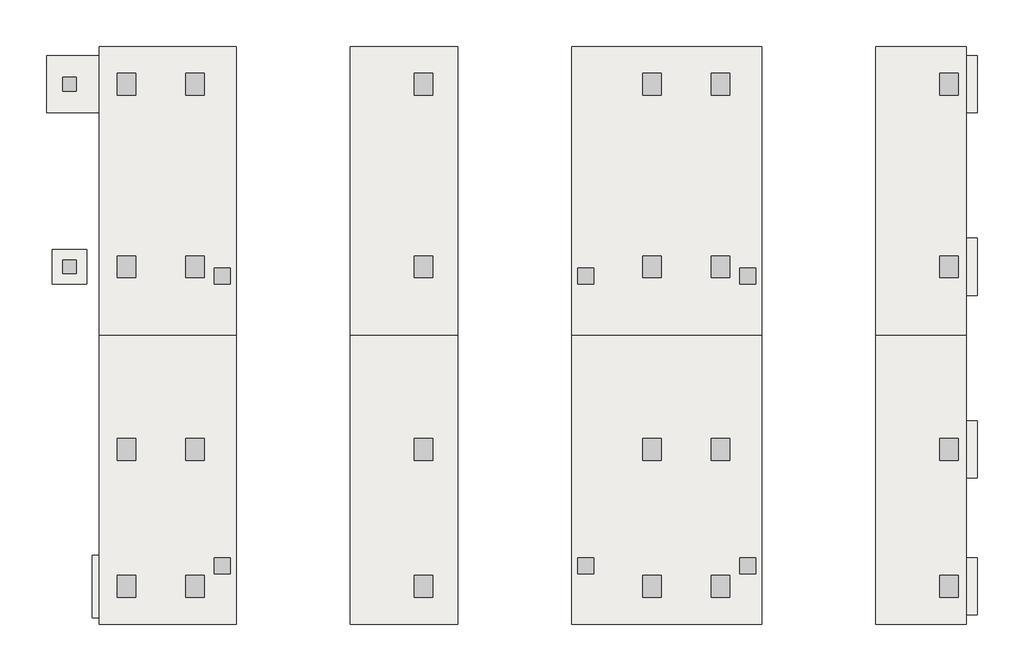
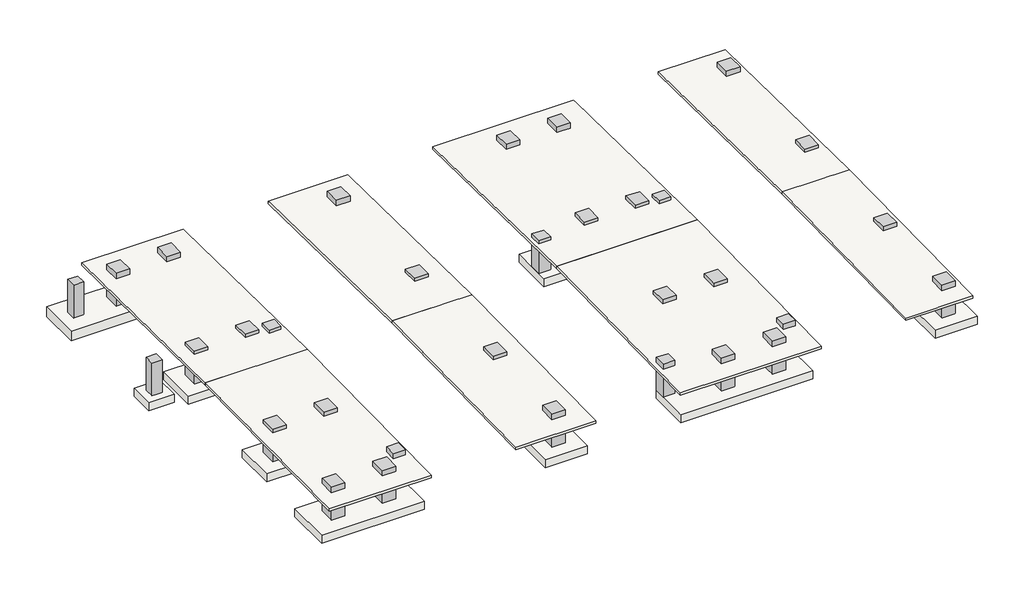
# Not in any storey: 32 columns, 25 slabs.
"""IFC4 building model written with IfcOpenShell, lengths in millimetres."""

import ifcopenshell
import ifcopenshell.guid

model = None  # the IFC model being written
_history = None  # IfcOwnerHistory: only IFC2X3 demands one
_inside = {}  # id of a spatial element -> (the spatial element, [elements in it])
_under = {}  # id of a project, library or spatial element -> (it, [spatial elements below it])
_declared = {}  # id of a project -> (the project, [libraries it declares])
_typed = {}  # id of a type object -> (the type object, [elements of that type])
_made_of = {}  # id of a material, layer set ... -> (it, [elements and type objects made of it])


def new_model(schema):
    """Start an empty IFC model of exactly this schema.

    Asked for "IFC4X3", IfcOpenShell would pick the latest addendum, in which some entities
    have other attributes; the version numbers below select the first issue.
    IFC2X3 requires an IfcOwnerHistory on every rooted entity: one is made here for all.
    """
    global model, _history
    if schema == "IFC4X3":
        model = ifcopenshell.file(schema_version=(4, 3, 0, 0))
    else:
        model = ifcopenshell.file(schema=schema)
    _inside.clear()
    _under.clear()
    _declared.clear()
    _typed.clear()
    _made_of.clear()
    _history = None
    if model.schema == "IFC2X3":
        org = make("IfcOrganization", Name="unknown")
        user = make(
            "IfcPersonAndOrganization",
            ThePerson=make("IfcPerson", FamilyName="unknown"),
            TheOrganization=org,
        )
        app = make(
            "IfcApplication",
            ApplicationDeveloper=org,
            Version="unknown",
            ApplicationFullName="unknown",
            ApplicationIdentifier="unknown",
        )
        _history = make(
            "IfcOwnerHistory",
            OwningUser=user,
            OwningApplication=app,
            ChangeAction="ADDED",
            CreationDate=0,
        )
    return model


def make(cls, **values):
    """One entity of the class cls with the attributes given. An attribute that is None is left unset."""
    return model.create_entity(
        cls, **{name: value for name, value in values.items() if value is not None}
    )


def rooted(cls, **values):
    """An entity with a GlobalId (a new one), such as an element, a storey or a relation."""
    return make(cls, GlobalId=ifcopenshell.guid.new(), OwnerHistory=_history, **values)


def si_unit(unit_type, name, prefix=None):
    """IfcSIUnit, for example si_unit("LENGTHUNIT", "METRE", prefix="MILLI")."""
    return make("IfcSIUnit", UnitType=unit_type, Prefix=prefix, Name=name)


def assignment(units):
    """IfcUnitAssignment: the units of a project."""
    return None if units is None else make("IfcUnitAssignment", Units=units)


def point(xyz):
    """IfcCartesianPoint."""
    return None if xyz is None else make("IfcCartesianPoint", Coordinates=xyz)


def direction(xyz):
    """IfcDirection."""
    return None if xyz is None else make("IfcDirection", DirectionRatios=xyz)


def frame(location, z_axis=None, x_axis=None):
    """IfcAxis2Placement3D, a coordinate frame: its origin and axes. An axis left out is left unset."""
    return make(
        "IfcAxis2Placement3D",
        Location=point(location),
        Axis=direction(z_axis),
        RefDirection=direction(x_axis),
    )


def origin():
    """The frame at (0, 0, 0) with its axes left unset."""
    return frame((0.0, 0.0, 0.0))


def place(relative_to, where):
    """IfcLocalPlacement: puts the frame where relative to a parent placement (None: the world)."""
    return make(
        "IfcLocalPlacement", PlacementRelTo=relative_to, RelativePlacement=where
    )


def context(
    kind, dimensions, precision=None, world=None, true_north=None, identifier=None
):
    """IfcGeometricRepresentationContext, for example the 3D "Model" context."""
    return make(
        "IfcGeometricRepresentationContext",
        ContextIdentifier=identifier,
        ContextType=kind,
        CoordinateSpaceDimension=dimensions,
        Precision=precision,
        WorldCoordinateSystem=world,
        TrueNorth=true_north,
    )


def project(units=None, contexts=None):
    """IfcProject with its units and contexts."""
    return rooted(
        "IfcProject",
        Name="project",
        RepresentationContexts=contexts,
        UnitsInContext=assignment(units),
    )


def spatial(cls, under=None, at=None, **own):
    """A site, building, storey or space (cls), placed at a placement, below another one or the project."""
    s = rooted(cls, ObjectPlacement=at, **own)
    if under is not None:
        _under.setdefault(under.id(), (under, []))[1].append(s)
    return s


def polyline(points):
    """IfcPolyline through the points."""
    return make("IfcPolyline", Points=[point(p) for p in points])


def outline(outer, holes=None, kind="AREA"):
    """IfcArbitraryClosedProfileDef: a profile drawn as a closed curve; with holes, ...WithVoids."""
    if holes is None:
        return make("IfcArbitraryClosedProfileDef", ProfileType=kind, OuterCurve=outer)
    return make(
        "IfcArbitraryProfileDefWithVoids",
        ProfileType=kind,
        OuterCurve=outer,
        InnerCurves=holes,
    )


def extrude(swept, where, along, depth):
    """IfcExtrudedAreaSolid: the profile swept, set in the frame where, extruded along a direction by depth."""
    return make(
        "IfcExtrudedAreaSolid",
        SweptArea=swept,
        Position=where,
        ExtrudedDirection=direction(along),
        Depth=depth,
    )


def faces_of(points, faces, orient=None, outer=None):
    """IfcFace entities. A face is a list of loops; a loop is a list of indices into points, from 0.

    orient and outer hold one flag for each loop. By default every Orientation is true, the
    first loop of a face is its IfcFaceOuterBound and the others are IfcFaceBound.
    """
    made = []
    for i, loops in enumerate(faces):
        bounds = []
        for j, loop in enumerate(loops):
            is_outer = j == 0 if outer is None else outer[i][j]
            bounds.append(
                make(
                    "IfcFaceOuterBound" if is_outer else "IfcFaceBound",
                    Bound=make("IfcPolyLoop", Polygon=[points[k] for k in loop]),
                    Orientation=True if orient is None else orient[i][j],
                )
            )
        made.append(make("IfcFace", Bounds=bounds))
    return made


def faceted_brep(points, faces, orient=None, outer=None, voids=None):
    """IfcFacetedBrep: a solid bounded by flat faces; with voids (closed shells), ...WithVoids."""
    shared = [point(p) for p in points]
    hull = make("IfcClosedShell", CfsFaces=faces_of(shared, faces, orient, outer))
    if voids is None:
        return make("IfcFacetedBrep", Outer=hull)
    return make(
        "IfcFacetedBrepWithVoids",
        Outer=hull,
        Voids=[
            make(cls, CfsFaces=faces_of(shared, fs, o, b)) for cls, fs, o, b in voids
        ],
    )


def shape(context_of_items, identifier, shape_type, items):
    """IfcShapeRepresentation: the items that make up one representation, for example the "Body"."""
    return make(
        "IfcShapeRepresentation",
        ContextOfItems=context_of_items,
        RepresentationIdentifier=identifier,
        RepresentationType=shape_type,
        Items=items,
    )


def source(mapping_origin, context_of_items, identifier, shape_type, items):
    """IfcRepresentationMap: a shape defined once, which mapped items show again and again."""
    return make(
        "IfcRepresentationMap",
        MappingOrigin=mapping_origin,
        MappedRepresentation=shape(context_of_items, identifier, shape_type, items),
    )


def transform(
    local_origin,
    x_axis=None,
    y_axis=None,
    z_axis=None,
    scale=None,
    scale2=None,
    scale3=None,
    uniform=True,
):
    """IfcCartesianTransformationOperator3D, or its non-uniform kind. x_axis, y_axis, z_axis: its Axis1, 2, 3."""
    if uniform:
        return make(
            "IfcCartesianTransformationOperator3D",
            Axis1=direction(x_axis),
            Axis2=direction(y_axis),
            LocalOrigin=point(local_origin),
            Scale=scale,
            Axis3=direction(z_axis),
        )
    return make(
        "IfcCartesianTransformationOperator3DnonUniform",
        Axis1=direction(x_axis),
        Axis2=direction(y_axis),
        LocalOrigin=point(local_origin),
        Scale=scale,
        Axis3=direction(z_axis),
        Scale2=scale2,
        Scale3=scale3,
    )


def mapped(mapping_source, mapping_target):
    """IfcMappedItem: shows the shape of a source again, moved by a transform."""
    return make(
        "IfcMappedItem", MappingSource=mapping_source, MappingTarget=mapping_target
    )


def made_of(thing, what):
    """Note that an element or type object is made of a material, layer set ...; save() writes the relation."""
    if what is not None:
        _made_of.setdefault(what.id(), (what, []))[1].append(thing)
    return thing


def element(
    cls,
    number,
    at=None,
    inside=None,
    cuts=None,
    type_object=None,
    material=None,
    context=None,
    identifier="Body",
    shape_type=None,
    held_by="IfcProductDefinitionShape",
    body=None,
    shapes=None,
    **own,
):
    """One element of the class cls, such as IfcWall. Its Tag is "e" and its number.

    at: its placement. inside: the storey or other place that contains it. cuts: it is an
    opening in that element (IfcRelVoidsElement). A single representation is given by context,
    identifier, shape_type and body (its items); several are given by shapes. held_by: the class
    of the entity that holds the representations. save() writes the other relations.
    """
    e = rooted(cls, Tag="e%d" % number, ObjectPlacement=at, **own)
    if body is not None:
        shapes = [shape(context, identifier, shape_type, body)]
    if shapes is not None:
        e.Representation = make(held_by, Representations=shapes)
    if inside is not None:
        _inside.setdefault(inside.id(), (inside, []))[1].append(e)
    if cuts is not None:
        rooted(
            "IfcRelVoidsElement", RelatingBuildingElement=cuts, RelatedOpeningElement=e
        )
    if type_object is not None:
        _typed.setdefault(type_object.id(), (type_object, []))[1].append(e)
    return made_of(e, material)


def aggregate(whole, parts):
    """IfcRelAggregates: a whole, such as a stair, and the parts it consists of."""
    return rooted("IfcRelAggregates", RelatingObject=whole, RelatedObjects=parts)


def save(model, path):
    """Write the relations noted so far, then the file.

    IfcRelAggregates (storeys below a building ...), IfcRelContainedInSpatialStructure (elements
    in a storey), IfcRelDefinesByType, IfcRelAssociatesMaterial and IfcRelDeclares: one each for
    every whole, place, type object, material and project.
    """
    for whole, parts in _under.values():
        aggregate(whole, parts)
    for where, things in _inside.values():
        rooted(
            "IfcRelContainedInSpatialStructure",
            RelatedElements=things,
            RelatingStructure=where,
        )
    for kind, things in _typed.values():
        rooted("IfcRelDefinesByType", RelatedObjects=things, RelatingType=kind)
    for what, things in _made_of.values():
        rooted("IfcRelAssociatesMaterial", RelatedObjects=things, RelatingMaterial=what)
    for by, libraries in _declared.values():
        rooted("IfcRelDeclares", RelatingContext=by, RelatedDefinitions=libraries)
    model.write(path)


def rc_column_rectangular_8fcc3407(model_context):
    return source(origin(), model_context, "Body", "SweptSolid", [
        extrude(outline(polyline([(400.0, 475.0), (400.0, -475.0), (-400.0, -475.0), (-400.0, 475.0), (400.0, 475.0)])), frame((0.0, 0.0, -9380.1756499), z_axis=(0.0, 0.0, 1.0), x_axis=(1.0, 0.0, 0.0)), (0.0, 0.0, 1.0), 2050.0),
    ])


def rc_column_rectangular_fa199b6f(model_context):
    return source(origin(), model_context, "Body", "SweptSolid", [
        extrude(outline(polyline([(300.0, 300.0), (300.0, -300.0), (-300.0, -300.0), (-300.0, 300.0), (300.0, 300.0)])), frame((0.0, 0.0, -9380.1756499), z_axis=(0.0, 0.0, 1.0), x_axis=(1.0, 0.0, 0.0)), (0.0, 0.0, 1.0), 2050.0),
    ])


def rc_column_rectangular_f0532c4b(model_context):
    return source(origin(), model_context, "Body", "SweptSolid", [
        extrude(outline(polyline([(350.0, 350.0), (350.0, -350.0), (-350.0, -350.0), (-350.0, 350.0), (350.0, 350.0)])), frame((0.0, 0.0, -9380.1756499), z_axis=(0.0, 0.0, 1.0), x_axis=(1.0, 0.0, 0.0)), (0.0, 0.0, 1.0), 2050.0),
    ])


def footing_rectangular_r1_513089b3(model_context):
    return source(origin(), model_context, "Body", "SweptSolid", [
        extrude(outline(polyline([(1250.0, 1250.0), (1250.0, -1250.0), (-1250.0, -1250.0), (-1250.0, 1250.0), (1250.0, 1250.0)])), frame((0.0, 0.0, -500.0), z_axis=(0.0, 0.0, 1.0), x_axis=(1.0, 0.0, 0.0)), (0.0, 0.0, 1.0), 500.0),
    ])


def footing_rectangular_r1_601d9235(model_context):
    return source(origin(), model_context, "Body", "SweptSolid", [
        extrude(outline(polyline([(750.0, 750.0), (750.0, -750.0), (-750.0, -750.0), (-750.0, 750.0), (750.0, 750.0)])), frame((0.0, 0.0, -500.0), z_axis=(0.0, 0.0, 1.0), x_axis=(1.0, 0.0, 0.0)), (0.0, 0.0, 1.0), 500.0),
    ])


def footing_rectangular_r1_ca059662(model_context):
    return source(origin(), model_context, "Body", "SweptSolid", [
        extrude(outline(polyline([(2700.0, 1250.0), (2700.0, -1250.0), (-2700.0, -1250.0), (-2700.0, 1250.0), (2700.0, 1250.0)])), frame((0.0, 0.0, -500.0), z_axis=(0.0, 0.0, 1.0), x_axis=(1.0, 0.0, 0.0)), (0.0, 0.0, 1.0), 500.0),
    ])


def footing_rectangular_r1_297981ed(model_context):
    return source(origin(), model_context, "Body", "SweptSolid", [
        extrude(outline(polyline([(3000.0, 1250.0), (3000.0, -1250.0), (-3000.0, -1250.0), (-3000.0, 1250.0), (3000.0, 1250.0)])), frame((0.0, 0.0, -500.0), z_axis=(0.0, 0.0, 1.0), x_axis=(1.0, 0.0, 0.0)), (0.0, 0.0, 1.0), 500.0),
    ])


def footing_rectangular_r1_282b4f06(model_context):
    return source(origin(), model_context, "Body", "SweptSolid", [
        extrude(outline(polyline([(4000.0, 1250.0), (4000.0, -1250.0), (-4000.0, -1250.0), (-4000.0, 1250.0), (4000.0, 1250.0)])), frame((0.0, 0.0, -600.0), z_axis=(0.0, 0.0, 1.0), x_axis=(1.0, 0.0, 0.0)), (0.0, 0.0, 1.0), 600.0),
    ])


def footing_rectangular_r1_f7e30f5b(model_context):
    return source(origin(), model_context, "Body", "SweptSolid", [
        extrude(outline(polyline([(2875.0, 1250.0), (2875.0, -1250.0), (-2875.0, -1250.0), (-2875.0, 1250.0), (2875.0, 1250.0)])), frame((0.0, 0.0, -500.0), z_axis=(0.0, 0.0, 1.0), x_axis=(1.0, 0.0, 0.0)), (0.0, 0.0, 1.0), 500.0),
    ])


def footing_rectangular_r1_e1557040(model_context):
    return source(origin(), model_context, "Body", "SweptSolid", [
        extrude(outline(polyline([(3900.0, 1250.0), (3900.0, -1250.0), (-3900.0, -1250.0), (-3900.0, 1250.0), (3900.0, 1250.0)])), frame((0.0, 0.0, -500.0), z_axis=(0.0, 0.0, 1.0), x_axis=(1.0, 0.0, 0.0)), (0.0, 0.0, 1.0), 500.0),
    ])


def footing_rectangular_r1_8e80394c(model_context):
    return source(origin(), model_context, "Body", "SweptSolid", [
        extrude(outline(polyline([(3025.0, 1370.0), (3025.0, -1370.0), (-3025.0, -1370.0), (-3025.0, 1370.0), (3025.0, 1370.0)])), frame((0.0, 0.0, -500.0), z_axis=(0.0, 0.0, 1.0), x_axis=(1.0, 0.0, 0.0)), (0.0, 0.0, 1.0), 500.0),
    ])


model = new_model("IFC4")

# Units and contexts
model_context = context("Model", 3, world=origin())
ifc_project = project(units=[si_unit("LENGTHUNIT", "METRE", prefix="MILLI")], contexts=[model_context])

# Site, building
site = spatial("IfcSite", under=ifc_project)
building = spatial("IfcBuilding", under=site)

# Columns
placement = place(None, origin())
rc_column_rectangular_shape = rc_column_rectangular_8fcc3407(model_context)
element("IfcColumn", 1, ObjectType="RC_Column_Rectangular : H_SC_AR_S15_UG PED_W800xL950_Bit_PD1", at=placement, inside=building, context=model_context, shape_type="MappedRepresentation", body=[
    mapped(rc_column_rectangular_shape, transform((36000.0, 499.5208589, 0.0), x_axis=(1.0, 0.0, 0.0), y_axis=(0.0, 1.0, 0.0), z_axis=(0.0, 0.0, 1.0))),
])
element("IfcColumn", 2, ObjectType="RC_Column_Rectangular : H_SC_AR_S15_UG PED_W800xL950_Bit_PD1", at=placement, inside=building, context=model_context, shape_type="MappedRepresentation", body=[
    mapped(rc_column_rectangular_shape, transform((36000.0, 6499.5208589, 0.0), x_axis=(1.0, 0.0, 0.0), y_axis=(0.0, 1.0, 0.0), z_axis=(0.0, 0.0, 1.0))),
])
element("IfcColumn", 3, ObjectType="RC_Column_Rectangular : H_SC_AR_S15_UG PED_W800xL950_Bit_PD1", at=placement, inside=building, context=model_context, shape_type="MappedRepresentation", body=[
    mapped(rc_column_rectangular_shape, transform((36000.0, 14499.5208589, 0.0), x_axis=(1.0, 0.0, 0.0), y_axis=(0.0, 1.0, 0.0), z_axis=(0.0, 0.0, 1.0))),
])
element("IfcColumn", 4, ObjectType="RC_Column_Rectangular : H_SC_AR_S15_UG PED_W800xL950_Bit_PD1", at=placement, inside=building, context=model_context, shape_type="MappedRepresentation", body=[
    mapped(rc_column_rectangular_shape, transform((36000.0, 22499.5208589, 0.0), x_axis=(1.0, 0.0, 0.0), y_axis=(0.0, 1.0, 0.0), z_axis=(0.0, 0.0, 1.0))),
])
element("IfcColumn", 5, ObjectType="RC_Column_Rectangular : H_SC_AR_S15_UG PED_W800xL950_Bit_PD1", at=placement, inside=building, context=model_context, shape_type="MappedRepresentation", body=[
    mapped(rc_column_rectangular_shape, transform((26000.0, 499.5208589, 0.0), x_axis=(1.0, 0.0, 0.0), y_axis=(0.0, 1.0, 0.0), z_axis=(0.0, 0.0, 1.0))),
])
element("IfcColumn", 6, ObjectType="RC_Column_Rectangular : H_SC_AR_S15_UG PED_W800xL950_Bit_PD1", at=placement, inside=building, context=model_context, shape_type="MappedRepresentation", body=[
    mapped(rc_column_rectangular_shape, transform((26000.0, 6499.5208589, 0.0), x_axis=(1.0, 0.0, 0.0), y_axis=(0.0, 1.0, 0.0), z_axis=(0.0, 0.0, 1.0))),
])
element("IfcColumn", 7, ObjectType="RC_Column_Rectangular : H_SC_AR_S15_UG PED_W800xL950_Bit_PD1", at=placement, inside=building, context=model_context, shape_type="MappedRepresentation", body=[
    mapped(rc_column_rectangular_shape, transform((26000.0, 14499.5208589, 0.0), x_axis=(1.0, 0.0, 0.0), y_axis=(0.0, 1.0, 0.0), z_axis=(0.0, 0.0, 1.0))),
])
element("IfcColumn", 8, ObjectType="RC_Column_Rectangular : H_SC_AR_S15_UG PED_W800xL950_Bit_PD1", at=placement, inside=building, context=model_context, shape_type="MappedRepresentation", body=[
    mapped(rc_column_rectangular_shape, transform((26000.0, 22499.5208589, 0.0), x_axis=(1.0, 0.0, 0.0), y_axis=(0.0, 1.0, 0.0), z_axis=(0.0, 0.0, 1.0))),
])
element("IfcColumn", 9, ObjectType="RC_Column_Rectangular : H_SC_AR_S15_UG PED_W800xL950_Bit_PD1", at=placement, inside=building, context=model_context, shape_type="MappedRepresentation", body=[
    mapped(rc_column_rectangular_shape, transform((23000.0, 499.5208589, 0.0), x_axis=(1.0, 0.0, 0.0), y_axis=(0.0, 1.0, 0.0), z_axis=(0.0, 0.0, 1.0))),
])
element("IfcColumn", 10, ObjectType="RC_Column_Rectangular : H_SC_AR_S15_UG PED_W800xL950_Bit_PD1", at=placement, inside=building, context=model_context, shape_type="MappedRepresentation", body=[
    mapped(rc_column_rectangular_shape, transform((23000.0, 6499.5208589, 0.0), x_axis=(1.0, 0.0, 0.0), y_axis=(0.0, 1.0, 0.0), z_axis=(0.0, 0.0, 1.0))),
])
element("IfcColumn", 11, ObjectType="RC_Column_Rectangular : H_SC_AR_S15_UG PED_W800xL950_Bit_PD1", at=placement, inside=building, context=model_context, shape_type="MappedRepresentation", body=[
    mapped(rc_column_rectangular_shape, transform((23000.0, 14499.5208589, 0.0), x_axis=(1.0, 0.0, 0.0), y_axis=(0.0, 1.0, 0.0), z_axis=(0.0, 0.0, 1.0))),
])
element("IfcColumn", 12, ObjectType="RC_Column_Rectangular : H_SC_AR_S15_UG PED_W800xL950_Bit_PD1", at=placement, inside=building, context=model_context, shape_type="MappedRepresentation", body=[
    mapped(rc_column_rectangular_shape, transform((23000.0, 22499.5208589, 0.0), x_axis=(1.0, 0.0, 0.0), y_axis=(0.0, 1.0, 0.0), z_axis=(0.0, 0.0, 1.0))),
])
element("IfcColumn", 13, ObjectType="RC_Column_Rectangular : H_SC_AR_S15_UG PED_W800xL950_Bit_PD1", at=placement, inside=building, context=model_context, shape_type="MappedRepresentation", body=[
    mapped(rc_column_rectangular_shape, transform((13000.0, 499.5208589, 0.0), x_axis=(1.0, 0.0, 0.0), y_axis=(0.0, 1.0, 0.0), z_axis=(0.0, 0.0, 1.0))),
])
element("IfcColumn", 14, ObjectType="RC_Column_Rectangular : H_SC_AR_S15_UG PED_W800xL950_Bit_PD1", at=placement, inside=building, context=model_context, shape_type="MappedRepresentation", body=[
    mapped(rc_column_rectangular_shape, transform((13000.0, 6499.5208589, 0.0), x_axis=(1.0, 0.0, 0.0), y_axis=(0.0, 1.0, 0.0), z_axis=(0.0, 0.0, 1.0))),
])
element("IfcColumn", 15, ObjectType="RC_Column_Rectangular : H_SC_AR_S15_UG PED_W800xL950_Bit_PD1", at=placement, inside=building, context=model_context, shape_type="MappedRepresentation", body=[
    mapped(rc_column_rectangular_shape, transform((13000.0, 14499.5208589, 0.0), x_axis=(1.0, 0.0, 0.0), y_axis=(0.0, 1.0, 0.0), z_axis=(0.0, 0.0, 1.0))),
])
element("IfcColumn", 16, ObjectType="RC_Column_Rectangular : H_SC_AR_S15_UG PED_W800xL950_Bit_PD1", at=placement, inside=building, context=model_context, shape_type="MappedRepresentation", body=[
    mapped(rc_column_rectangular_shape, transform((13000.0, 22499.5208589, 0.0), x_axis=(1.0, 0.0, 0.0), y_axis=(0.0, 1.0, 0.0), z_axis=(0.0, 0.0, 1.0))),
])
element("IfcColumn", 17, ObjectType="RC_Column_Rectangular : H_SC_AR_S15_UG PED_W800xL950_Bit_PD1", at=placement, inside=building, context=model_context, shape_type="MappedRepresentation", body=[
    mapped(rc_column_rectangular_shape, transform((3000.0, 499.5208589, 0.0), x_axis=(1.0, 0.0, 0.0), y_axis=(0.0, 1.0, 0.0), z_axis=(0.0, 0.0, 1.0))),
])
element("IfcColumn", 18, ObjectType="RC_Column_Rectangular : H_SC_AR_S15_UG PED_W800xL950_Bit_PD1", at=placement, inside=building, context=model_context, shape_type="MappedRepresentation", body=[
    mapped(rc_column_rectangular_shape, transform((3000.0, 6499.5208589, 0.0), x_axis=(1.0, 0.0, 0.0), y_axis=(0.0, 1.0, 0.0), z_axis=(0.0, 0.0, 1.0))),
])
element("IfcColumn", 19, ObjectType="RC_Column_Rectangular : H_SC_AR_S15_UG PED_W800xL950_Bit_PD1", at=placement, inside=building, context=model_context, shape_type="MappedRepresentation", body=[
    mapped(rc_column_rectangular_shape, transform((3000.0, 14499.5208589, 0.0), x_axis=(1.0, 0.0, 0.0), y_axis=(0.0, 1.0, 0.0), z_axis=(0.0, 0.0, 1.0))),
])
element("IfcColumn", 20, ObjectType="RC_Column_Rectangular : H_SC_AR_S15_UG PED_W800xL950_Bit_PD1", at=placement, inside=building, context=model_context, shape_type="MappedRepresentation", body=[
    mapped(rc_column_rectangular_shape, transform((3000.0, 22499.5208589, 0.0), x_axis=(1.0, 0.0, 0.0), y_axis=(0.0, 1.0, 0.0), z_axis=(0.0, 0.0, 1.0))),
])
element("IfcColumn", 21, ObjectType="RC_Column_Rectangular : H_SC_AR_S15_UG PED_W800xL950_Bit_PD1", at=placement, inside=building, context=model_context, shape_type="MappedRepresentation", body=[
    mapped(rc_column_rectangular_shape, transform((0.0, 499.5208589, 0.0), x_axis=(1.0, 0.0, 0.0), y_axis=(0.0, 1.0, 0.0), z_axis=(0.0, 0.0, 1.0))),
])
element("IfcColumn", 22, ObjectType="RC_Column_Rectangular : H_SC_AR_S15_UG PED_W800xL950_Bit_PD1", at=placement, inside=building, context=model_context, shape_type="MappedRepresentation", body=[
    mapped(rc_column_rectangular_shape, transform((0.0, 6499.5208589, 0.0), x_axis=(1.0, 0.0, 0.0), y_axis=(0.0, 1.0, 0.0), z_axis=(0.0, 0.0, 1.0))),
])
element("IfcColumn", 23, ObjectType="RC_Column_Rectangular : H_SC_AR_S15_UG PED_W800xL950_Bit_PD1", at=placement, inside=building, context=model_context, shape_type="MappedRepresentation", body=[
    mapped(rc_column_rectangular_shape, transform((0.0, 14499.5208589, 0.0), x_axis=(1.0, 0.0, 0.0), y_axis=(0.0, 1.0, 0.0), z_axis=(0.0, 0.0, 1.0))),
])
element("IfcColumn", 24, ObjectType="RC_Column_Rectangular : H_SC_AR_S15_UG PED_W800xL950_Bit_PD1", at=placement, inside=building, context=model_context, shape_type="MappedRepresentation", body=[
    mapped(rc_column_rectangular_shape, transform((0.0, 22499.5208589, 0.0), x_axis=(1.0, 0.0, 0.0), y_axis=(0.0, 1.0, 0.0), z_axis=(0.0, 0.0, 1.0))),
])
rc_column_rectangular_2_shape = rc_column_rectangular_fa199b6f(model_context)
element("IfcColumn", 25, ObjectType="RC_Column_Rectangular : H_SC_AR_S15_UG PED_W600xL600_Bit_PD2", at=placement, inside=building, context=model_context, shape_type="MappedRepresentation", body=[
    mapped(rc_column_rectangular_2_shape, transform((-2500.0, 22499.5208589, 0.0), x_axis=(1.0, 0.0, 0.0), y_axis=(0.0, 1.0, 0.0), z_axis=(0.0, 0.0, 1.0))),
])
element("IfcColumn", 26, ObjectType="RC_Column_Rectangular : H_SC_AR_S15_UG PED_W600xL600_Bit_PD2", at=placement, inside=building, context=model_context, shape_type="MappedRepresentation", body=[
    mapped(rc_column_rectangular_2_shape, transform((-2500.0, 14499.5208589, 0.0), x_axis=(1.0, 0.0, 0.0), y_axis=(0.0, 1.0, 0.0), z_axis=(0.0, 0.0, 1.0))),
])
rc_column_rectangular_3_shape = rc_column_rectangular_f0532c4b(model_context)
element("IfcColumn", 27, ObjectType="RC_Column_Rectangular : H_SC_AR_S15_UG PED_W700xL700_Bit_PD3", at=placement, inside=building, context=model_context, shape_type="MappedRepresentation", body=[
    mapped(rc_column_rectangular_3_shape, transform((4200.0, 1399.5208589, 0.0), x_axis=(1.0, 0.0, 0.0), y_axis=(0.0, 1.0, 0.0), z_axis=(0.0, 0.0, 1.0))),
])
element("IfcColumn", 28, ObjectType="RC_Column_Rectangular : H_SC_AR_S15_UG PED_W700xL700_Bit_PD3", at=placement, inside=building, context=model_context, shape_type="MappedRepresentation", body=[
    mapped(rc_column_rectangular_3_shape, transform((27200.0, 1399.5208589, 0.0), x_axis=(1.0, 0.0, 0.0), y_axis=(0.0, 1.0, 0.0), z_axis=(0.0, 0.0, 1.0))),
])
element("IfcColumn", 29, ObjectType="RC_Column_Rectangular : H_SC_AR_S15_UG PED_W700xL700_Bit_PD3", at=placement, inside=building, context=model_context, shape_type="MappedRepresentation", body=[
    mapped(rc_column_rectangular_3_shape, transform((20100.0, 1399.5208589, 0.0), x_axis=(1.0, 0.0, 0.0), y_axis=(0.0, 1.0, 0.0), z_axis=(0.0, 0.0, 1.0))),
])
element("IfcColumn", 30, ObjectType="RC_Column_Rectangular : H_SC_AR_S15_UG PED_W700xL700_Bit_PD3", at=placement, inside=building, context=model_context, shape_type="MappedRepresentation", body=[
    mapped(rc_column_rectangular_3_shape, transform((4200.0, 14099.5208589, 0.0), x_axis=(1.0, 0.0, 0.0), y_axis=(0.0, 1.0, 0.0), z_axis=(0.0, 0.0, 1.0))),
])
element("IfcColumn", 31, ObjectType="RC_Column_Rectangular : H_SC_AR_S15_UG PED_W700xL700_Bit_PD3", at=placement, inside=building, context=model_context, shape_type="MappedRepresentation", body=[
    mapped(rc_column_rectangular_3_shape, transform((27200.0, 14099.5208589, 0.0), x_axis=(1.0, 0.0, 0.0), y_axis=(0.0, 1.0, 0.0), z_axis=(0.0, 0.0, 1.0))),
])
element("IfcColumn", 32, ObjectType="RC_Column_Rectangular : H_SC_AR_S15_UG PED_W700xL700_Bit_PD3", at=placement, inside=building, context=model_context, shape_type="MappedRepresentation", body=[
    mapped(rc_column_rectangular_3_shape, transform((20100.0, 14099.5208589, 0.0), x_axis=(1.0, 0.0, 0.0), y_axis=(0.0, 1.0, 0.0), z_axis=(0.0, 0.0, 1.0))),
])

# Slabs
element("IfcSlab", 33, ObjectType="H_SF_AR_S17_SOG T150", at=placement, inside=building, context=model_context, shape_type="Brep", body=[
    faceted_brep([(32800.0, 11499.5208589, -7630.1943961), (36750.0, 11499.5208589, -7630.1943961), (36750.0, -1150.4791411, -7830.1943961), (32800.0, -1150.4791411, -7830.1943961), (36400.0, 6974.5208589, -7701.7358981), (35600.0, 6974.5208589, -7701.7358981), (35600.0, 6024.5208589, -7716.7556609), (36400.0, 6024.5208589, -7716.7556609), (36400.0, 974.5208589, -7796.5975581), (35600.0, 974.5208589, -7796.5975581), (35600.0, 24.5208589, -7811.617321), (36400.0, 24.5208589, -7811.617321), (32800.0, 11499.5208589, -7480.1756499), (32800.0, -950.4791411, -7677.0135946), (32800.0, -1150.4791411, -7680.1756499), (36550.0, -1150.4791411, -7680.1756499), (36750.0, -1150.4791411, -7680.1756499), (36750.0, 11499.5208589, -7480.1756499), (36400.0, 6974.5208589, -7551.7171519), (36400.0, 6024.5208589, -7566.7369147), (35600.0, 6024.5208589, -7566.7369147), (35600.0, 6974.5208589, -7551.7171519), (36400.0, 974.5208589, -7646.5788119), (36400.0, 24.5208589, -7661.5985748), (35600.0, 24.5208589, -7661.5985748), (35600.0, 974.5208589, -7646.5788119)], [[[0, 1, 2, 3], [4, 5, 6, 7], [8, 9, 10, 11]], [[12, 13, 14, 15, 16, 17], [18, 19, 20, 21], [22, 23, 24, 25]], [[2, 1, 17, 16]], [[3, 2, 16, 15, 14]], [[0, 3, 14, 13, 12]], [[5, 4, 18, 21]], [[6, 5, 21, 20]], [[7, 6, 20, 19]], [[4, 7, 19, 18]], [[9, 8, 22, 25]], [[10, 9, 25, 24]], [[11, 10, 24, 23]], [[8, 11, 23, 22]], [[1, 0, 12, 17]]]),
])
element("IfcSlab", 34, ObjectType="H_SF_AR_S17_SOG T150", at=placement, inside=building, context=model_context, shape_type="Brep", body=[
    faceted_brep([(19500.0, 11499.5208589, -7630.1943961), (27800.0, 11499.5208589, -7630.1943961), (27800.0, -1150.4791411, -7830.1943961), (19500.0, -1150.4791411, -7830.1943961), (20450.0, 1049.5208589, -7795.4117874), (20450.0, 1749.5208589, -7784.3445937), (19750.0, 1749.5208589, -7784.3445937), (19750.0, 1049.5208589, -7795.4117874), (23400.0, 974.5208589, -7796.5975581), (22600.0, 974.5208589, -7796.5975581), (22600.0, 24.5208589, -7811.617321), (23400.0, 24.5208589, -7811.617321), (26400.0, 24.5208589, -7811.617321), (26400.0, 974.5208589, -7796.5975581), (25600.0, 974.5208589, -7796.5975581), (25600.0, 24.5208589, -7811.617321), (27550.0, 1749.5208589, -7784.3445937), (26850.0, 1749.5208589, -7784.3445937), (26850.0, 1049.5208589, -7795.4117874), (27550.0, 1049.5208589, -7795.4117874), (25600.0, 6024.5208589, -7716.7556609), (26400.0, 6024.5208589, -7716.7556609), (26400.0, 6974.5208589, -7701.7358981), (25600.0, 6974.5208589, -7701.7358981), (23400.0, 6974.5208589, -7701.7358981), (22600.0, 6974.5208589, -7701.7358981), (22600.0, 6024.5208589, -7716.7556609), (23400.0, 6024.5208589, -7716.7556609), (19500.0, 11499.5208589, -7480.1756499), (19500.0, -950.4791411, -7677.0135946), (19500.0, -1150.4791411, -7680.1756499), (27800.0, -1150.4791411, -7680.1756499), (27800.0, -950.4791411, -7677.0135946), (27800.0, 11499.5208589, -7480.1756499), (20450.0, 1049.5208589, -7645.3930412), (19750.0, 1049.5208589, -7645.3930412), (19750.0, 1749.5208589, -7634.3258475), (20450.0, 1749.5208589, -7634.3258475), (23400.0, 974.5208589, -7646.5788119), (23400.0, 24.5208589, -7661.5985748), (22600.0, 24.5208589, -7661.5985748), (22600.0, 974.5208589, -7646.5788119), (26400.0, 24.5208589, -7661.5985748), (25600.0, 24.5208589, -7661.5985748), (25600.0, 974.5208589, -7646.5788119), (26400.0, 974.5208589, -7646.5788119), (27550.0, 1749.5208589, -7634.3258475), (27550.0, 1049.5208589, -7645.3930412), (26850.0, 1049.5208589, -7645.3930412), (26850.0, 1749.5208589, -7634.3258475), (25600.0, 6024.5208589, -7566.7369147), (25600.0, 6974.5208589, -7551.7171519), (26400.0, 6974.5208589, -7551.7171519), (26400.0, 6024.5208589, -7566.7369147), (23400.0, 6974.5208589, -7551.7171519), (23400.0, 6024.5208589, -7566.7369147), (22600.0, 6024.5208589, -7566.7369147), (22600.0, 6974.5208589, -7551.7171519)], [[[0, 1, 2, 3], [4, 5, 6, 7], [8, 9, 10, 11], [12, 13, 14, 15], [16, 17, 18, 19], [20, 21, 22, 23], [24, 25, 26, 27]], [[28, 29, 30, 31, 32, 33], [34, 35, 36, 37], [38, 39, 40, 41], [42, 43, 44, 45], [46, 47, 48, 49], [50, 51, 52, 53], [54, 55, 56, 57]], [[1, 0, 28, 33]], [[2, 1, 33, 32, 31]], [[3, 2, 31, 30]], [[0, 3, 30, 29, 28]], [[5, 4, 34, 37]], [[6, 5, 37, 36]], [[7, 6, 36, 35]], [[4, 7, 35, 34]], [[9, 8, 38, 41]], [[10, 9, 41, 40]], [[11, 10, 40, 39]], [[8, 11, 39, 38]], [[13, 12, 42, 45]], [[14, 13, 45, 44]], [[15, 14, 44, 43]], [[12, 15, 43, 42]], [[17, 16, 46, 49]], [[18, 17, 49, 48]], [[19, 18, 48, 47]], [[16, 19, 47, 46]], [[21, 20, 50, 53]], [[22, 21, 53, 52]], [[23, 22, 52, 51]], [[20, 23, 51, 50]], [[25, 24, 54, 57]], [[26, 25, 57, 56]], [[27, 26, 56, 55]], [[24, 27, 55, 54]]]),
])
element("IfcSlab", 35, ObjectType="H_SF_AR_S17_SOG T150", at=placement, inside=building, context=model_context, shape_type="Brep", body=[
    faceted_brep([(27800.0, 11499.5208589, -7630.1943961), (19500.0, 11499.5208589, -7630.1943961), (19500.0, 24149.5208589, -7830.1943961), (27800.0, 24149.5208589, -7830.1943961), (19750.0, 13749.5208589, -7665.7675186), (20450.0, 13749.5208589, -7665.7675186), (20450.0, 14449.5208589, -7676.8347123), (19750.0, 14449.5208589, -7676.8347123), (23400.0, 14024.5208589, -7670.1153447), (23400.0, 14974.5208589, -7685.1351075), (22600.0, 14974.5208589, -7685.1351075), (22600.0, 14024.5208589, -7670.1153447), (26400.0, 14974.5208589, -7685.1351075), (25600.0, 14974.5208589, -7685.1351075), (25600.0, 14024.5208589, -7670.1153447), (26400.0, 14024.5208589, -7670.1153447), (27550.0, 13749.5208589, -7665.7675186), (27550.0, 14449.5208589, -7676.8347123), (26850.0, 14449.5208589, -7676.8347123), (26850.0, 13749.5208589, -7665.7675186), (26400.0, 22024.5208589, -7796.5975581), (26400.0, 22974.5208589, -7811.617321), (25600.0, 22974.5208589, -7811.617321), (25600.0, 22024.5208589, -7796.5975581), (22600.0, 22024.5208589, -7796.5975581), (23400.0, 22024.5208589, -7796.5975581), (23400.0, 22974.5208589, -7811.617321), (22600.0, 22974.5208589, -7811.617321), (27800.0, 11499.5208589, -7480.1756499), (27800.0, 23949.5208589, -7677.0135946), (27800.0, 24149.5208589, -7680.1756499), (19500.0, 24149.5208589, -7680.1756499), (19500.0, 23949.5208589, -7677.0135946), (19500.0, 11499.5208589, -7480.1756499), (19750.0, 13749.5208589, -7515.7487724), (19750.0, 14449.5208589, -7526.8159661), (20450.0, 14449.5208589, -7526.8159661), (20450.0, 13749.5208589, -7515.7487724), (23400.0, 14024.5208589, -7520.0965985), (22600.0, 14024.5208589, -7520.0965985), (22600.0, 14974.5208589, -7535.1163614), (23400.0, 14974.5208589, -7535.1163614), (26400.0, 14974.5208589, -7535.1163614), (26400.0, 14024.5208589, -7520.0965985), (25600.0, 14024.5208589, -7520.0965985), (25600.0, 14974.5208589, -7535.1163614), (27550.0, 13749.5208589, -7515.7487724), (26850.0, 13749.5208589, -7515.7487724), (26850.0, 14449.5208589, -7526.8159661), (27550.0, 14449.5208589, -7526.8159661), (26400.0, 22024.5208589, -7646.5788119), (25600.0, 22024.5208589, -7646.5788119), (25600.0, 22974.5208589, -7661.5985748), (26400.0, 22974.5208589, -7661.5985748), (22600.0, 22024.5208589, -7646.5788119), (22600.0, 22974.5208589, -7661.5985748), (23400.0, 22974.5208589, -7661.5985748), (23400.0, 22024.5208589, -7646.5788119)], [[[0, 1, 2, 3], [4, 5, 6, 7], [8, 9, 10, 11], [12, 13, 14, 15], [16, 17, 18, 19], [20, 21, 22, 23], [24, 25, 26, 27]], [[28, 29, 30, 31, 32, 33], [34, 35, 36, 37], [38, 39, 40, 41], [42, 43, 44, 45], [46, 47, 48, 49], [50, 51, 52, 53], [54, 55, 56, 57]], [[1, 0, 28, 33]], [[2, 1, 33, 32, 31]], [[3, 2, 31, 30]], [[0, 3, 30, 29, 28]], [[5, 4, 34, 37]], [[6, 5, 37, 36]], [[7, 6, 36, 35]], [[4, 7, 35, 34]], [[9, 8, 38, 41]], [[10, 9, 41, 40]], [[11, 10, 40, 39]], [[8, 11, 39, 38]], [[13, 12, 42, 45]], [[14, 13, 45, 44]], [[15, 14, 44, 43]], [[12, 15, 43, 42]], [[17, 16, 46, 49]], [[18, 17, 49, 48]], [[19, 18, 48, 47]], [[16, 19, 47, 46]], [[21, 20, 50, 53]], [[22, 21, 53, 52]], [[23, 22, 52, 51]], [[20, 23, 51, 50]], [[25, 24, 54, 57]], [[26, 25, 57, 56]], [[27, 26, 56, 55]], [[24, 27, 55, 54]]]),
])
element("IfcSlab", 36, ObjectType="H_SF_AR_S17_SOG T150", at=placement, inside=building, context=model_context, shape_type="Brep", body=[
    faceted_brep([(36750.0, 24149.5208589, -7830.1943961), (36750.0, 11499.5208589, -7630.1943961), (32800.0, 11499.5208589, -7630.1943961), (32800.0, 24149.5208589, -7830.1943961), (36400.0, 22974.5208589, -7811.617321), (35600.0, 22974.5208589, -7811.617321), (35600.0, 22024.5208589, -7796.5975581), (36400.0, 22024.5208589, -7796.5975581), (35600.0, 14024.5208589, -7670.1153447), (36400.0, 14024.5208589, -7670.1153447), (36400.0, 14974.5208589, -7685.1351075), (35600.0, 14974.5208589, -7685.1351075), (36750.0, 24149.5208589, -7680.1756499), (32800.0, 24149.5208589, -7680.1756499), (32800.0, 23949.5208589, -7677.0135946), (32800.0, 11499.5208589, -7480.1756499), (36750.0, 11499.5208589, -7480.1756499), (36750.0, 23949.5208589, -7677.0135946), (36400.0, 22974.5208589, -7661.5985748), (36400.0, 22024.5208589, -7646.5788119), (35600.0, 22024.5208589, -7646.5788119), (35600.0, 22974.5208589, -7661.5985748), (35600.0, 14024.5208589, -7520.0965985), (35600.0, 14974.5208589, -7535.1163614), (36400.0, 14974.5208589, -7535.1163614), (36400.0, 14024.5208589, -7520.0965985)], [[[0, 1, 2, 3], [4, 5, 6, 7], [8, 9, 10, 11]], [[12, 13, 14, 15, 16, 17], [18, 19, 20, 21], [22, 23, 24, 25]], [[1, 0, 12, 17, 16]], [[2, 1, 16, 15]], [[3, 2, 15, 14, 13]], [[0, 3, 13, 12]], [[5, 4, 18, 21]], [[6, 5, 21, 20]], [[7, 6, 20, 19]], [[4, 7, 19, 18]], [[9, 8, 22, 25]], [[10, 9, 25, 24]], [[11, 10, 24, 23]], [[8, 11, 23, 22]]]),
])
element("IfcSlab", 37, ObjectType="H_SF_AR_S17_SOG T150", at=placement, inside=building, context=model_context, shape_type="Brep", body=[
    faceted_brep([(9800.0, 11499.5208589, -7630.1943961), (14500.0, 11499.5208589, -7630.1943961), (14500.0, -1150.4791411, -7830.1943961), (9800.0, -1150.4791411, -7830.1943961), (13400.0, 6974.5208589, -7701.7358981), (12600.0, 6974.5208589, -7701.7358981), (12600.0, 6024.5208589, -7716.7556609), (13400.0, 6024.5208589, -7716.7556609), (13400.0, 974.5208589, -7796.5975581), (12600.0, 974.5208589, -7796.5975581), (12600.0, 24.5208589, -7811.617321), (13400.0, 24.5208589, -7811.617321), (9800.0, 11499.5208589, -7480.1756499), (9800.0, -950.4791411, -7677.0135946), (9800.0, -1150.4791411, -7680.1756499), (14500.0, -1150.4791411, -7680.1756499), (14500.0, -950.4791411, -7677.0135946), (14500.0, 11499.5208589, -7480.1756499), (13400.0, 6974.5208589, -7551.7171519), (13400.0, 6024.5208589, -7566.7369147), (12600.0, 6024.5208589, -7566.7369147), (12600.0, 6974.5208589, -7551.7171519), (13400.0, 974.5208589, -7646.5788119), (13400.0, 24.5208589, -7661.5985748), (12600.0, 24.5208589, -7661.5985748), (12600.0, 974.5208589, -7646.5788119)], [[[0, 1, 2, 3], [4, 5, 6, 7], [8, 9, 10, 11]], [[12, 13, 14, 15, 16, 17], [18, 19, 20, 21], [22, 23, 24, 25]], [[2, 1, 17, 16, 15]], [[3, 2, 15, 14]], [[0, 3, 14, 13, 12]], [[5, 4, 18, 21]], [[6, 5, 21, 20]], [[7, 6, 20, 19]], [[4, 7, 19, 18]], [[9, 8, 22, 25]], [[10, 9, 25, 24]], [[11, 10, 24, 23]], [[8, 11, 23, 22]], [[1, 0, 12, 17]]]),
])
element("IfcSlab", 38, ObjectType="H_SF_AR_S17_SOG T150", at=placement, inside=building, context=model_context, shape_type="Brep", body=[
    faceted_brep([(14500.0, 24149.5208589, -7830.1943961), (14500.0, 11499.5208589, -7630.1943961), (9800.0, 11499.5208589, -7630.1943961), (9800.0, 24149.5208589, -7830.1943961), (13400.0, 22974.5208589, -7811.617321), (12600.0, 22974.5208589, -7811.617321), (12600.0, 22024.5208589, -7796.5975581), (13400.0, 22024.5208589, -7796.5975581), (12600.0, 14024.5208589, -7670.1153447), (13400.0, 14024.5208589, -7670.1153447), (13400.0, 14974.5208589, -7685.1351075), (12600.0, 14974.5208589, -7685.1351075), (14500.0, 24149.5208589, -7680.1756499), (9800.0, 24149.5208589, -7680.1756499), (9800.0, 23949.5208589, -7677.0135946), (9800.0, 11499.5208589, -7480.1756499), (14500.0, 11499.5208589, -7480.1756499), (14500.0, 23949.5208589, -7677.0135946), (13400.0, 22974.5208589, -7661.5985748), (13400.0, 22024.5208589, -7646.5788119), (12600.0, 22024.5208589, -7646.5788119), (12600.0, 22974.5208589, -7661.5985748), (12600.0, 14024.5208589, -7520.0965985), (12600.0, 14974.5208589, -7535.1163614), (13400.0, 14974.5208589, -7535.1163614), (13400.0, 14024.5208589, -7520.0965985)], [[[0, 1, 2, 3], [4, 5, 6, 7], [8, 9, 10, 11]], [[12, 13, 14, 15, 16, 17], [18, 19, 20, 21], [22, 23, 24, 25]], [[1, 0, 12, 17, 16]], [[2, 1, 16, 15]], [[3, 2, 15, 14, 13]], [[0, 3, 13, 12]], [[5, 4, 18, 21]], [[6, 5, 21, 20]], [[7, 6, 20, 19]], [[4, 7, 19, 18]], [[9, 8, 22, 25]], [[10, 9, 25, 24]], [[11, 10, 24, 23]], [[8, 11, 23, 22]]]),
])
element("IfcSlab", 39, ObjectType="H_SF_AR_S17_SOG T150", at=placement, inside=building, context=model_context, shape_type="Brep", body=[
    faceted_brep([(-1200.0, 11499.5208589, -7630.1943961), (4800.0, 11499.5208589, -7630.1943961), (4800.0, -1150.4791411, -7830.1943961), (-1200.0, -1150.4791411, -7830.1943961), (400.0, 974.5208589, -7796.5975581), (-400.0, 974.5208589, -7796.5975581), (-400.0, 24.5208589, -7811.617321), (400.0, 24.5208589, -7811.617321), (3400.0, 24.5208589, -7811.617321), (3400.0, 974.5208589, -7796.5975581), (2600.0, 974.5208589, -7796.5975581), (2600.0, 24.5208589, -7811.617321), (4550.0, 1749.5208589, -7784.3445937), (3850.0, 1749.5208589, -7784.3445937), (3850.0, 1049.5208589, -7795.4117874), (4550.0, 1049.5208589, -7795.4117874), (2600.0, 6024.5208589, -7716.7556609), (3400.0, 6024.5208589, -7716.7556609), (3400.0, 6974.5208589, -7701.7358981), (2600.0, 6974.5208589, -7701.7358981), (400.0, 6974.5208589, -7701.7358981), (-400.0, 6974.5208589, -7701.7358981), (-400.0, 6024.5208589, -7716.7556609), (400.0, 6024.5208589, -7716.7556609), (-1200.0, 11499.5208589, -7480.1756499), (-1200.0, -950.4791411, -7677.0135946), (-1200.0, -1150.4791411, -7680.1756499), (4800.0, -1150.4791411, -7680.1756499), (4800.0, -950.4791411, -7677.0135946), (4800.0, 11499.5208589, -7480.1756499), (400.0, 974.5208589, -7646.5788119), (400.0, 24.5208589, -7661.5985748), (-400.0, 24.5208589, -7661.5985748), (-400.0, 974.5208589, -7646.5788119), (3400.0, 24.5208589, -7661.5985748), (2600.0, 24.5208589, -7661.5985748), (2600.0, 974.5208589, -7646.5788119), (3400.0, 974.5208589, -7646.5788119), (4550.0, 1749.5208589, -7634.3258475), (4550.0, 1049.5208589, -7645.3930412), (3850.0, 1049.5208589, -7645.3930412), (3850.0, 1749.5208589, -7634.3258475), (2600.0, 6024.5208589, -7566.7369147), (2600.0, 6974.5208589, -7551.7171519), (3400.0, 6974.5208589, -7551.7171519), (3400.0, 6024.5208589, -7566.7369147), (400.0, 6974.5208589, -7551.7171519), (400.0, 6024.5208589, -7566.7369147), (-400.0, 6024.5208589, -7566.7369147), (-400.0, 6974.5208589, -7551.7171519)], [[[0, 1, 2, 3], [4, 5, 6, 7], [8, 9, 10, 11], [12, 13, 14, 15], [16, 17, 18, 19], [20, 21, 22, 23]], [[24, 25, 26, 27, 28, 29], [30, 31, 32, 33], [34, 35, 36, 37], [38, 39, 40, 41], [42, 43, 44, 45], [46, 47, 48, 49]], [[1, 0, 24, 29]], [[2, 1, 29, 28, 27]], [[3, 2, 27, 26]], [[0, 3, 26, 25, 24]], [[5, 4, 30, 33]], [[6, 5, 33, 32]], [[7, 6, 32, 31]], [[4, 7, 31, 30]], [[9, 8, 34, 37]], [[10, 9, 37, 36]], [[11, 10, 36, 35]], [[8, 11, 35, 34]], [[13, 12, 38, 41]], [[14, 13, 41, 40]], [[15, 14, 40, 39]], [[12, 15, 39, 38]], [[17, 16, 42, 45]], [[18, 17, 45, 44]], [[19, 18, 44, 43]], [[16, 19, 43, 42]], [[21, 20, 46, 49]], [[22, 21, 49, 48]], [[23, 22, 48, 47]], [[20, 23, 47, 46]]]),
])
element("IfcSlab", 40, ObjectType="H_SF_AR_S17_SOG T150", at=placement, inside=building, context=model_context, shape_type="Brep", body=[
    faceted_brep([(4800.0, 11499.5208589, -7630.1943961), (-1200.0, 11499.5208589, -7630.1943961), (-1200.0, 24149.5208589, -7830.1943961), (4800.0, 24149.5208589, -7830.1943961), (400.0, 14024.5208589, -7670.1153447), (400.0, 14974.5208589, -7685.1351075), (-400.0, 14974.5208589, -7685.1351075), (-400.0, 14024.5208589, -7670.1153447), (3400.0, 14974.5208589, -7685.1351075), (2600.0, 14974.5208589, -7685.1351075), (2600.0, 14024.5208589, -7670.1153447), (3400.0, 14024.5208589, -7670.1153447), (4550.0, 13749.5208589, -7665.7675186), (4550.0, 14449.5208589, -7676.8347123), (3850.0, 14449.5208589, -7676.8347123), (3850.0, 13749.5208589, -7665.7675186), (3400.0, 22024.5208589, -7796.5975581), (3400.0, 22974.5208589, -7811.617321), (2600.0, 22974.5208589, -7811.617321), (2600.0, 22024.5208589, -7796.5975581), (-400.0, 22024.5208589, -7796.5975581), (400.0, 22024.5208589, -7796.5975581), (400.0, 22974.5208589, -7811.617321), (-400.0, 22974.5208589, -7811.617321), (4800.0, 11499.5208589, -7480.1756499), (4800.0, 23949.5208589, -7677.0135946), (4800.0, 24149.5208589, -7680.1756499), (-1200.0, 24149.5208589, -7680.1756499), (-1200.0, 23949.5208589, -7677.0135946), (-1200.0, 11499.5208589, -7480.1756499), (400.0, 14024.5208589, -7520.0965985), (-400.0, 14024.5208589, -7520.0965985), (-400.0, 14974.5208589, -7535.1163614), (400.0, 14974.5208589, -7535.1163614), (3400.0, 14974.5208589, -7535.1163614), (3400.0, 14024.5208589, -7520.0965985), (2600.0, 14024.5208589, -7520.0965985), (2600.0, 14974.5208589, -7535.1163614), (4550.0, 13749.5208589, -7515.7487724), (3850.0, 13749.5208589, -7515.7487724), (3850.0, 14449.5208589, -7526.8159661), (4550.0, 14449.5208589, -7526.8159661), (3400.0, 22024.5208589, -7646.5788119), (2600.0, 22024.5208589, -7646.5788119), (2600.0, 22974.5208589, -7661.5985748), (3400.0, 22974.5208589, -7661.5985748), (-400.0, 22024.5208589, -7646.5788119), (-400.0, 22974.5208589, -7661.5985748), (400.0, 22974.5208589, -7661.5985748), (400.0, 22024.5208589, -7646.5788119)], [[[0, 1, 2, 3], [4, 5, 6, 7], [8, 9, 10, 11], [12, 13, 14, 15], [16, 17, 18, 19], [20, 21, 22, 23]], [[24, 25, 26, 27, 28, 29], [30, 31, 32, 33], [34, 35, 36, 37], [38, 39, 40, 41], [42, 43, 44, 45], [46, 47, 48, 49]], [[1, 0, 24, 29]], [[2, 1, 29, 28, 27]], [[3, 2, 27, 26]], [[0, 3, 26, 25, 24]], [[5, 4, 30, 33]], [[6, 5, 33, 32]], [[7, 6, 32, 31]], [[4, 7, 31, 30]], [[9, 8, 34, 37]], [[10, 9, 37, 36]], [[11, 10, 36, 35]], [[8, 11, 35, 34]], [[13, 12, 38, 41]], [[14, 13, 41, 40]], [[15, 14, 40, 39]], [[12, 15, 39, 38]], [[17, 16, 42, 45]], [[18, 17, 45, 44]], [[19, 18, 44, 43]], [[16, 19, 43, 42]], [[21, 20, 46, 49]], [[22, 21, 49, 48]], [[23, 22, 48, 47]], [[20, 23, 47, 46]]]),
])
footing_rectangular_r1_shape = footing_rectangular_r1_513089b3(model_context)
element("IfcSlab", 41, ObjectType="Footing-Rectangular_R1 : H_SF_AR_S18_W2500xL2500xT500_Bitumen_F1", at=placement, inside=building, context=model_context, shape_type="MappedRepresentation", body=[
    mapped(footing_rectangular_r1_shape, transform((13000.0, 22499.5208589, -9380.1756499), x_axis=(1.0, 0.0, 0.0), y_axis=(0.0, 1.0, 0.0), z_axis=(0.0, 0.0, 1.0))),
])
element("IfcSlab", 42, ObjectType="Footing-Rectangular_R1 : H_SF_AR_S18_W2500xL2500xT500_Bitumen_F1", at=placement, inside=building, context=model_context, shape_type="MappedRepresentation", body=[
    mapped(footing_rectangular_r1_shape, transform((13000.0, 14499.5208589, -9380.1756499), x_axis=(1.0, 0.0, 0.0), y_axis=(0.0, 1.0, 0.0), z_axis=(0.0, 0.0, 1.0))),
])
element("IfcSlab", 43, ObjectType="Footing-Rectangular_R1 : H_SF_AR_S18_W2500xL2500xT500_Bitumen_F1", at=placement, inside=building, context=model_context, shape_type="MappedRepresentation", body=[
    mapped(footing_rectangular_r1_shape, transform((13000.0, 6499.5208589, -9380.1756499), x_axis=(1.0, 0.0, 0.0), y_axis=(0.0, 1.0, 0.0), z_axis=(0.0, 0.0, 1.0))),
])
element("IfcSlab", 44, ObjectType="Footing-Rectangular_R1 : H_SF_AR_S18_W2500xL2500xT500_Bitumen_F1", at=placement, inside=building, context=model_context, shape_type="MappedRepresentation", body=[
    mapped(footing_rectangular_r1_shape, transform((13000.0, 499.5208589, -9380.1756499), x_axis=(1.0, 0.0, 0.0), y_axis=(0.0, 1.0, 0.0), z_axis=(0.0, 0.0, 1.0))),
])
element("IfcSlab", 45, ObjectType="Footing-Rectangular_R1 : H_SF_AR_S18_W2500xL2500xT500_Bitumen_F1", at=placement, inside=building, context=model_context, shape_type="MappedRepresentation", body=[
    mapped(footing_rectangular_r1_shape, transform((36000.0, 22499.5208589, -9380.1756499), x_axis=(1.0, 0.0, 0.0), y_axis=(0.0, 1.0, 0.0), z_axis=(0.0, 0.0, 1.0))),
])
element("IfcSlab", 46, ObjectType="Footing-Rectangular_R1 : H_SF_AR_S18_W2500xL2500xT500_Bitumen_F1", at=placement, inside=building, context=model_context, shape_type="MappedRepresentation", body=[
    mapped(footing_rectangular_r1_shape, transform((36000.0, 14499.5208589, -9380.1756499), x_axis=(1.0, 0.0, 0.0), y_axis=(0.0, 1.0, 0.0), z_axis=(0.0, 0.0, 1.0))),
])
element("IfcSlab", 47, ObjectType="Footing-Rectangular_R1 : H_SF_AR_S18_W2500xL2500xT500_Bitumen_F1", at=placement, inside=building, context=model_context, shape_type="MappedRepresentation", body=[
    mapped(footing_rectangular_r1_shape, transform((36000.0, 6499.5208589, -9380.1756499), x_axis=(1.0, 0.0, 0.0), y_axis=(0.0, 1.0, 0.0), z_axis=(0.0, 0.0, 1.0))),
])
element("IfcSlab", 48, ObjectType="Footing-Rectangular_R1 : H_SF_AR_S18_W2500xL2500xT500_Bitumen_F1", at=placement, inside=building, context=model_context, shape_type="MappedRepresentation", body=[
    mapped(footing_rectangular_r1_shape, transform((36000.0, 499.5208589, -9380.1756499), x_axis=(1.0, 0.0, 0.0), y_axis=(0.0, 1.0, 0.0), z_axis=(0.0, 0.0, 1.0))),
])
footing_rectangular_r1_2_shape = footing_rectangular_r1_601d9235(model_context)
element("IfcSlab", 49, ObjectType="Footing-Rectangular_R1 : H_SF_AR_S18_W1500xL1500xT500_Bitumen_F2", at=placement, inside=building, context=model_context, shape_type="MappedRepresentation", body=[
    mapped(footing_rectangular_r1_2_shape, transform((-2500.0, 14499.5208589, -9380.1756499), x_axis=(1.0, 0.0, 0.0), y_axis=(0.0, 1.0, 0.0), z_axis=(0.0, 0.0, 1.0))),
])
footing_rectangular_r1_3_shape = footing_rectangular_r1_ca059662(model_context)
element("IfcSlab", 50, ObjectType="Footing-Rectangular_R1 : H_SF_AR_S18_W5400xL2500xT500_Bitumen_F3", at=placement, inside=building, context=model_context, shape_type="MappedRepresentation", body=[
    mapped(footing_rectangular_r1_3_shape, transform((24500.0, 6499.5208589, -9380.1756499), x_axis=(1.0, 0.0, 0.0), y_axis=(0.0, 1.0, 0.0), z_axis=(0.0, 0.0, 1.0))),
])
element("IfcSlab", 51, ObjectType="Footing-Rectangular_R1 : H_SF_AR_S18_W5400xL2500xT500_Bitumen_F3", at=placement, inside=building, context=model_context, shape_type="MappedRepresentation", body=[
    mapped(footing_rectangular_r1_3_shape, transform((1500.0, 6499.5208589, -9380.1756499), x_axis=(1.0, 0.0, 0.0), y_axis=(0.0, 1.0, 0.0), z_axis=(0.0, 0.0, 1.0))),
])
footing_rectangular_r1_4_shape = footing_rectangular_r1_297981ed(model_context)
element("IfcSlab", 52, ObjectType="Footing-Rectangular_R1 : H_SF_AR_S18_W6000xL2500xT500_Bitumen_F4", at=placement, inside=building, context=model_context, shape_type="MappedRepresentation", body=[
    mapped(footing_rectangular_r1_4_shape, transform((24500.0, 22499.5208589, -9380.1756499), x_axis=(1.0, 0.0, 0.0), y_axis=(0.0, 1.0, 0.0), z_axis=(0.0, 0.0, 1.0))),
])
footing_rectangular_r1_5_shape = footing_rectangular_r1_282b4f06(model_context)
element("IfcSlab", 53, ObjectType="Footing-Rectangular_R1 : H_SF_AR_S18_W8000xL2500xT500_Bitumen_F5", at=placement, inside=building, context=model_context, shape_type="MappedRepresentation", body=[
    mapped(footing_rectangular_r1_5_shape, transform((500.0, 22499.5208589, -9380.1756499), x_axis=(1.0, 0.0, 0.0), y_axis=(0.0, 1.0, 0.0), z_axis=(0.0, 0.0, 1.0))),
])
footing_rectangular_r1_6_shape = footing_rectangular_r1_f7e30f5b(model_context)
element("IfcSlab", 54, ObjectType="Footing-Rectangular_R1 : H_SF_AR_S18_W5750xL2500xT500_Bitumen_F6", at=placement, inside=building, context=model_context, shape_type="MappedRepresentation", body=[
    mapped(footing_rectangular_r1_6_shape, transform((1675.0, 14499.5208589, -9380.1756499), x_axis=(1.0, 0.0, 0.0), y_axis=(0.0, 1.0, 0.0), z_axis=(0.0, 0.0, 1.0))),
])
footing_rectangular_r1_7_shape = footing_rectangular_r1_e1557040(model_context)
element("IfcSlab", 55, ObjectType="Footing-Rectangular_R1 : H_SF_AR_S18_W7800xL2500xT500_Bitumen_F7", at=placement, inside=building, context=model_context, shape_type="MappedRepresentation", body=[
    mapped(footing_rectangular_r1_7_shape, transform((23650.0, 14499.5208589, -9380.1756499), x_axis=(1.0, 0.0, 0.0), y_axis=(0.0, 1.0, 0.0), z_axis=(0.0, 0.0, 1.0))),
])
footing_rectangular_r1_8_shape = footing_rectangular_r1_8e80394c(model_context)
element("IfcSlab", 56, ObjectType="Footing-Rectangular_R1 : H_SF_AR_S18_W6050xL2740xT500_Bitumen_F8", at=placement, inside=building, context=model_context, shape_type="MappedRepresentation", body=[
    mapped(footing_rectangular_r1_8_shape, transform((1525.0, 499.5208589, -9380.1756499), x_axis=(1.0, 0.0, 0.0), y_axis=(0.0, 1.0, 0.0), z_axis=(0.0, 0.0, 1.0))),
])
element("IfcSlab", 57, ObjectType="Footing-Rectangular_R1 : H_SF_AR_S18_W7800xL2740xT500_Bitumen_F9", at=placement, inside=building, context=model_context, shape_type="MappedRepresentation", body=[
    mapped(footing_rectangular_r1_7_shape, transform((23650.0, 499.5208589, -9380.1756499), x_axis=(1.0, 0.0, 0.0), y_axis=(0.0, 1.0, 0.0), z_axis=(0.0, 0.0, 1.0))),
])

save(model, "model.ifc")

# Revit data of these elements
# Type "RC_Column_Rectangular : H_SC_AR_S15_UG PED_W800xL950_Bit_PD1"
#   Type Mark = "PD1"
#   Width = 800 mm
#   Length = 950 mm
#   hec_material3 [instance default] = none
#   hec_material2 [instance default] = none
#   hec_material1 [instance default] = none
#   Structural Material [instance default] = none
#   Description = (empty or 0)
# Type "RC_Column_Rectangular : H_SC_AR_S15_UG PED_W600xL600_Bit_PD2"
#   Type Mark = "PD2"
#   Width = 600 mm
#   Length = 600 mm
#   hec_material3 [instance default] = none
#   hec_material2 [instance default] = none
#   hec_material1 [instance default] = none
#   Structural Material [instance default] = none
#   Description = (empty or 0)
# Type "RC_Column_Rectangular : H_SC_AR_S15_UG PED_W700xL700_Bit_PD3"
#   Type Mark = "PD3"
#   Width = 700 mm
#   Length = 700 mm
#   hec_material3 [instance default] = none
#   hec_material2 [instance default] = none
#   hec_material1 [instance default] = none
#   Structural Material [instance default] = none
#   Description = (empty or 0)
# Type "H_SF_AR_S17_SOG T150"
#   Type Comments = "구조_콘크리트"
#   Type Mark = "GS1"
#   Layers, outside or top first: 0 mm no material (function 100); 150 mm no material (function 1); 0 mm no material (function 100); 0 mm no material (function 100)
# Type "Footing-Rectangular_R1 : H_SF_AR_S18_W2500xL2500xT500_Bitumen_F1"
#   Type Mark = "F1"
#   Top bar = "D25@300"
#   Description = "UG Shallow Foundation"
#   Bottom bar = "D20@300"
#   Width = 2500 mm
#   Length = 2500 mm
#   Foundation Thickness = 500 mm
#   Structural Material [instance default] = none
#   Assembly Code = ""
# Type "Footing-Rectangular_R1 : H_SF_AR_S18_W1500xL1500xT500_Bitumen_F2"
#   Type Mark = "F2"
#   Top bar = "D25@300"
#   Description = "UG Shallow Foundation"
#   Bottom bar = "D20@300"
#   Width = 1500 mm
#   Length = 1500 mm
#   Foundation Thickness = 500 mm
#   Structural Material [instance default] = none
#   Assembly Code = ""
# Type "Footing-Rectangular_R1 : H_SF_AR_S18_W5400xL2500xT500_Bitumen_F3"
#   Type Mark = "F3"
#   Top bar = "D25@300"
#   Description = "UG Shallow Foundation"
#   Bottom bar = "D20@300"
#   Width = 5400 mm
#   Length = 2500 mm
#   Foundation Thickness = 500 mm
#   Structural Material [instance default] = none
#   Assembly Code = ""
# Type "Footing-Rectangular_R1 : H_SF_AR_S18_W6000xL2500xT500_Bitumen_F4"
#   Type Mark = "F4"
#   Top bar = "D25@300"
#   Description = "UG Shallow Foundation"
#   Bottom bar = "D20@300"
#   Width = 6000 mm
#   Length = 2500 mm
#   Foundation Thickness = 500 mm
#   Structural Material [instance default] = none
#   Assembly Code = ""
# Type "Footing-Rectangular_R1 : H_SF_AR_S18_W8000xL2500xT500_Bitumen_F5"
#   Type Mark = "F5"
#   Top bar = "D25@300"
#   Description = "UG Shallow Foundation"
#   Bottom bar = "D20@300"
#   Width = 8000 mm
#   Length = 2500 mm
#   Foundation Thickness = 600 mm
#   Structural Material [instance default] = none
#   Assembly Code = ""
# Type "Footing-Rectangular_R1 : H_SF_AR_S18_W5750xL2500xT500_Bitumen_F6"
#   Type Mark = "F6"
#   Top bar = "D25@300"
#   Description = "UG Shallow Foundation"
#   Bottom bar = "D20@300"
#   Width = 5750 mm
#   Length = 2500 mm
#   Foundation Thickness = 500 mm
#   Structural Material [instance default] = none
#   Assembly Code = ""
# Type "Footing-Rectangular_R1 : H_SF_AR_S18_W7800xL2500xT500_Bitumen_F7"
#   Type Mark = "F7"
#   Top bar = "D25@300"
#   Description = "UG Shallow Foundation"
#   Bottom bar = "D20@300"
#   Width = 7800 mm
#   Length = 2500 mm
#   Foundation Thickness = 500 mm
#   Structural Material [instance default] = none
#   Assembly Code = ""
# Type "Footing-Rectangular_R1 : H_SF_AR_S18_W6050xL2740xT500_Bitumen_F8"
#   Type Mark = "F8"
#   Top bar = "D25@300"
#   Description = "UG Shallow Foundation"
#   Bottom bar = "D20@300"
#   Width = 6050 mm
#   Length = 2740 mm
#   Foundation Thickness = 500 mm
#   Structural Material [instance default] = none
#   Assembly Code = ""
# Type "Footing-Rectangular_R1 : H_SF_AR_S18_W7800xL2740xT500_Bitumen_F9"
#   Type Mark = "F9"
#   Top bar = "D25@300"
#   Description = "UG Shallow Foundation"
#   Bottom bar = "D20@300"
